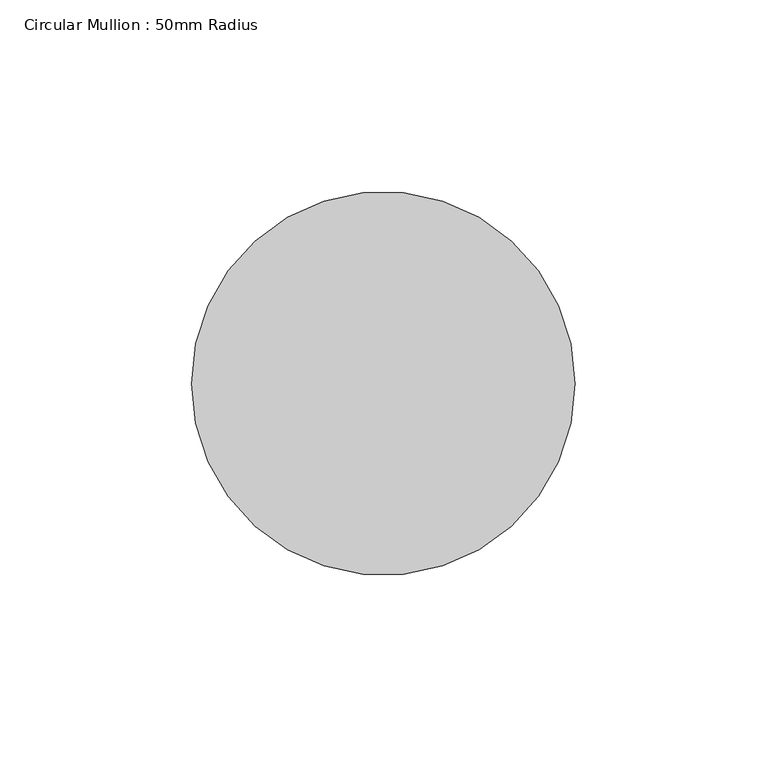
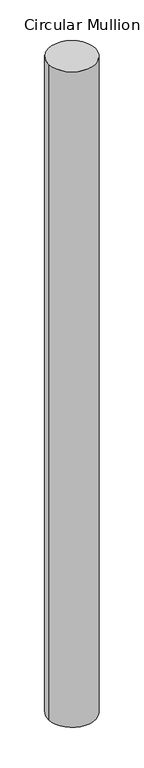
"""IFC4 building model written with IfcOpenShell, lengths in millimetres: member geometry, Circular Mullion : 50mm Radius."""

import ifcopenshell
import ifcopenshell.guid

model = None  # the IFC model being written
_history = None  # IfcOwnerHistory: only IFC2X3 demands one
_inside = {}  # id of a spatial element -> (the spatial element, [elements in it])
_under = {}  # id of a project, library or spatial element -> (it, [spatial elements below it])
_declared = {}  # id of a project -> (the project, [libraries it declares])
_typed = {}  # id of a type object -> (the type object, [elements of that type])
_made_of = {}  # id of a material, layer set ... -> (it, [elements and type objects made of it])


def new_model(schema):
    """Start an empty IFC model of exactly this schema.

    Asked for "IFC4X3", IfcOpenShell would pick the latest addendum, in which some entities
    have other attributes; the version numbers below select the first issue.
    IFC2X3 requires an IfcOwnerHistory on every rooted entity: one is made here for all.
    """
    global model, _history
    if schema == "IFC4X3":
        model = ifcopenshell.file(schema_version=(4, 3, 0, 0))
    else:
        model = ifcopenshell.file(schema=schema)
    _inside.clear()
    _under.clear()
    _declared.clear()
    _typed.clear()
    _made_of.clear()
    _history = None
    if model.schema == "IFC2X3":
        org = make("IfcOrganization", Name="unknown")
        user = make(
            "IfcPersonAndOrganization",
            ThePerson=make("IfcPerson", FamilyName="unknown"),
            TheOrganization=org,
        )
        app = make(
            "IfcApplication",
            ApplicationDeveloper=org,
            Version="unknown",
            ApplicationFullName="unknown",
            ApplicationIdentifier="unknown",
        )
        _history = make(
            "IfcOwnerHistory",
            OwningUser=user,
            OwningApplication=app,
            ChangeAction="ADDED",
            CreationDate=0,
        )
    return model


def make(cls, **values):
    """One entity of the class cls with the attributes given. An attribute that is None is left unset."""
    return model.create_entity(
        cls, **{name: value for name, value in values.items() if value is not None}
    )


def rooted(cls, **values):
    """An entity with a GlobalId (a new one), such as an element, a storey or a relation."""
    return make(cls, GlobalId=ifcopenshell.guid.new(), OwnerHistory=_history, **values)


def si_unit(unit_type, name, prefix=None):
    """IfcSIUnit, for example si_unit("LENGTHUNIT", "METRE", prefix="MILLI")."""
    return make("IfcSIUnit", UnitType=unit_type, Prefix=prefix, Name=name)


def assignment(units):
    """IfcUnitAssignment: the units of a project."""
    return None if units is None else make("IfcUnitAssignment", Units=units)


def point(xyz):
    """IfcCartesianPoint."""
    return None if xyz is None else make("IfcCartesianPoint", Coordinates=xyz)


def direction(xyz):
    """IfcDirection."""
    return None if xyz is None else make("IfcDirection", DirectionRatios=xyz)


def frame(location, z_axis=None, x_axis=None):
    """IfcAxis2Placement3D, a coordinate frame: its origin and axes. An axis left out is left unset."""
    return make(
        "IfcAxis2Placement3D",
        Location=point(location),
        Axis=direction(z_axis),
        RefDirection=direction(x_axis),
    )


def frame_2d(location, x_axis=None):
    """IfcAxis2Placement2D, a coordinate frame in the plane: its origin and x axis."""
    return make(
        "IfcAxis2Placement2D", Location=point(location), RefDirection=direction(x_axis)
    )


def origin():
    """The frame at (0, 0, 0) with its axes left unset."""
    return frame((0.0, 0.0, 0.0))


def origin_2d():
    """The frame at (0, 0) in the plane with its x axis left unset."""
    return frame_2d((0.0, 0.0))


def place(relative_to, where):
    """IfcLocalPlacement: puts the frame where relative to a parent placement (None: the world)."""
    return make(
        "IfcLocalPlacement", PlacementRelTo=relative_to, RelativePlacement=where
    )


def context(
    kind, dimensions, precision=None, world=None, true_north=None, identifier=None
):
    """IfcGeometricRepresentationContext, for example the 3D "Model" context."""
    return make(
        "IfcGeometricRepresentationContext",
        ContextIdentifier=identifier,
        ContextType=kind,
        CoordinateSpaceDimension=dimensions,
        Precision=precision,
        WorldCoordinateSystem=world,
        TrueNorth=true_north,
    )


def project(units=None, contexts=None):
    """IfcProject with its units and contexts."""
    return rooted(
        "IfcProject",
        Name="project",
        RepresentationContexts=contexts,
        UnitsInContext=assignment(units),
    )


def spatial(cls, under=None, at=None, **own):
    """A site, building, storey or space (cls), placed at a placement, below another one or the project."""
    s = rooted(cls, ObjectPlacement=at, **own)
    if under is not None:
        _under.setdefault(under.id(), (under, []))[1].append(s)
    return s


def circle_curve(where, radius):
    """IfcCircle in the frame where."""
    return make("IfcCircle", Position=where, Radius=radius)


def trimmed(basis, trim1, trim2, sense, master):
    """IfcTrimmedCurve: the piece of a basis curve between two trims."""
    return make(
        "IfcTrimmedCurve",
        BasisCurve=basis,
        Trim1=trim1,
        Trim2=trim2,
        SenseAgreement=sense,
        MasterRepresentation=master,
    )


def segment(curve, same_sense, transition):
    """IfcCompositeCurveSegment."""
    return make(
        "IfcCompositeCurveSegment",
        Transition=transition,
        SameSense=same_sense,
        ParentCurve=curve,
    )


def composite_curve(segments, self_intersect=None):
    """IfcCompositeCurve: segments joined end to end."""
    return make("IfcCompositeCurve", Segments=segments, SelfIntersect=self_intersect)


def outline(outer, holes=None, kind="AREA"):
    """IfcArbitraryClosedProfileDef: a profile drawn as a closed curve; with holes, ...WithVoids."""
    if holes is None:
        return make("IfcArbitraryClosedProfileDef", ProfileType=kind, OuterCurve=outer)
    return make(
        "IfcArbitraryProfileDefWithVoids",
        ProfileType=kind,
        OuterCurve=outer,
        InnerCurves=holes,
    )


def extrude(swept, where, along, depth):
    """IfcExtrudedAreaSolid: the profile swept, set in the frame where, extruded along a direction by depth."""
    return make(
        "IfcExtrudedAreaSolid",
        SweptArea=swept,
        Position=where,
        ExtrudedDirection=direction(along),
        Depth=depth,
    )


def shape(context_of_items, identifier, shape_type, items):
    """IfcShapeRepresentation: the items that make up one representation, for example the "Body"."""
    return make(
        "IfcShapeRepresentation",
        ContextOfItems=context_of_items,
        RepresentationIdentifier=identifier,
        RepresentationType=shape_type,
        Items=items,
    )


def source(mapping_origin, context_of_items, identifier, shape_type, items):
    """IfcRepresentationMap: a shape defined once, which mapped items show again and again."""
    return make(
        "IfcRepresentationMap",
        MappingOrigin=mapping_origin,
        MappedRepresentation=shape(context_of_items, identifier, shape_type, items),
    )


def transform(
    local_origin,
    x_axis=None,
    y_axis=None,
    z_axis=None,
    scale=None,
    scale2=None,
    scale3=None,
    uniform=True,
):
    """IfcCartesianTransformationOperator3D, or its non-uniform kind. x_axis, y_axis, z_axis: its Axis1, 2, 3."""
    if uniform:
        return make(
            "IfcCartesianTransformationOperator3D",
            Axis1=direction(x_axis),
            Axis2=direction(y_axis),
            LocalOrigin=point(local_origin),
            Scale=scale,
            Axis3=direction(z_axis),
        )
    return make(
        "IfcCartesianTransformationOperator3DnonUniform",
        Axis1=direction(x_axis),
        Axis2=direction(y_axis),
        LocalOrigin=point(local_origin),
        Scale=scale,
        Axis3=direction(z_axis),
        Scale2=scale2,
        Scale3=scale3,
    )


def mapped(mapping_source, mapping_target):
    """IfcMappedItem: shows the shape of a source again, moved by a transform."""
    return make(
        "IfcMappedItem", MappingSource=mapping_source, MappingTarget=mapping_target
    )


def made_of(thing, what):
    """Note that an element or type object is made of a material, layer set ...; save() writes the relation."""
    if what is not None:
        _made_of.setdefault(what.id(), (what, []))[1].append(thing)
    return thing


def element(
    cls,
    number,
    at=None,
    inside=None,
    cuts=None,
    type_object=None,
    material=None,
    context=None,
    identifier="Body",
    shape_type=None,
    held_by="IfcProductDefinitionShape",
    body=None,
    shapes=None,
    **own,
):
    """One element of the class cls, such as IfcWall. Its Tag is "e" and its number.

    at: its placement. inside: the storey or other place that contains it. cuts: it is an
    opening in that element (IfcRelVoidsElement). A single representation is given by context,
    identifier, shape_type and body (its items); several are given by shapes. held_by: the class
    of the entity that holds the representations. save() writes the other relations.
    """
    e = rooted(cls, Tag="e%d" % number, ObjectPlacement=at, **own)
    if body is not None:
        shapes = [shape(context, identifier, shape_type, body)]
    if shapes is not None:
        e.Representation = make(held_by, Representations=shapes)
    if inside is not None:
        _inside.setdefault(inside.id(), (inside, []))[1].append(e)
    if cuts is not None:
        rooted(
            "IfcRelVoidsElement", RelatingBuildingElement=cuts, RelatedOpeningElement=e
        )
    if type_object is not None:
        _typed.setdefault(type_object.id(), (type_object, []))[1].append(e)
    return made_of(e, material)


def aggregate(whole, parts):
    """IfcRelAggregates: a whole, such as a stair, and the parts it consists of."""
    return rooted("IfcRelAggregates", RelatingObject=whole, RelatedObjects=parts)


def save(model, path):
    """Write the relations noted so far, then the file.

    IfcRelAggregates (storeys below a building ...), IfcRelContainedInSpatialStructure (elements
    in a storey), IfcRelDefinesByType, IfcRelAssociatesMaterial and IfcRelDeclares: one each for
    every whole, place, type object, material and project.
    """
    for whole, parts in _under.values():
        aggregate(whole, parts)
    for where, things in _inside.values():
        rooted(
            "IfcRelContainedInSpatialStructure",
            RelatedElements=things,
            RelatingStructure=where,
        )
    for kind, things in _typed.values():
        rooted("IfcRelDefinesByType", RelatedObjects=things, RelatingType=kind)
    for what, things in _made_of.values():
        rooted("IfcRelAssociatesMaterial", RelatedObjects=things, RelatingMaterial=what)
    for by, libraries in _declared.values():
        rooted("IfcRelDeclares", RelatingContext=by, RelatedDefinitions=libraries)
    model.write(path)


def circular_mullion_50mm_radius_2b9c08a1(model_context):
    return source(origin(), model_context, "Body", "SweptSolid", [
        extrude(outline(composite_curve([segment(trimmed(circle_curve(origin_2d(), 50.0), [point((50.0, 0.0))], [point((-50.0, 0.0))], False, "CARTESIAN"), True, "CONTINUOUS"), segment(trimmed(circle_curve(origin_2d(), 50.0), [point((-50.0, 0.0))], [point((50.0, 0.0))], False, "CARTESIAN"), True, "CONTINUOUS")], self_intersect=False)), frame((0.0, 0.0, -1470.0014317), z_axis=(0.0, 0.0, 1.0), x_axis=(1.0, 0.0, 0.0)), (0.0, 0.0, 1.0), 1470.0014317),
    ])


if __name__ == "__main__":
    model = new_model("IFC4")
    model_context = context("Model", 3, world=origin())
    ifc_project = project(units=[si_unit("LENGTHUNIT", "METRE", prefix="MILLI")], contexts=[model_context])
    site = spatial("IfcSite", under=ifc_project)
    building = spatial("IfcBuilding", under=site)
    placement = place(None, origin())
    circular_mullion_50mm_radius_shape = circular_mullion_50mm_radius_2b9c08a1(model_context)
    element("IfcMember", 1, ObjectType="Circular Mullion : 50mm Radius", at=placement, inside=building, context=model_context, shape_type="MappedRepresentation", body=[
        mapped(circular_mullion_50mm_radius_shape, transform((0.0, 0.0, 0.0), x_axis=(1.0, 0.0, 0.0), y_axis=(0.0, 1.0, 0.0), z_axis=(0.0, 0.0, 1.0))),
    ])
    save(model, "model.ifc")

# Revit data of these elements
# Type "Circular Mullion : 50mm Radius"
#   built-in parameter 1007350 = 0.164042 (stored number, unit not read)
# Element 1 (IfcMember, "Circular Mullion : 50mm Radius")
#   Materials on its faces: "Aluminium"
# Materials
#   "Aluminium": class "Metal", colour RGB 247 247 247, transparency 0, Description = "Aluminium 6061", Cost = 0
